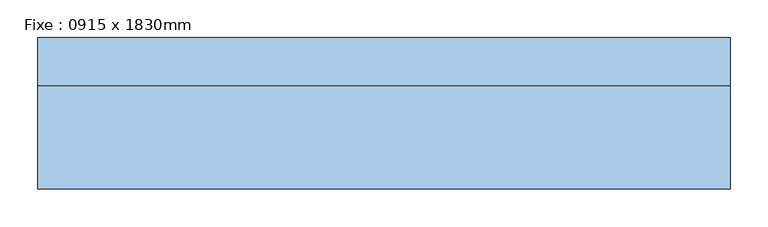
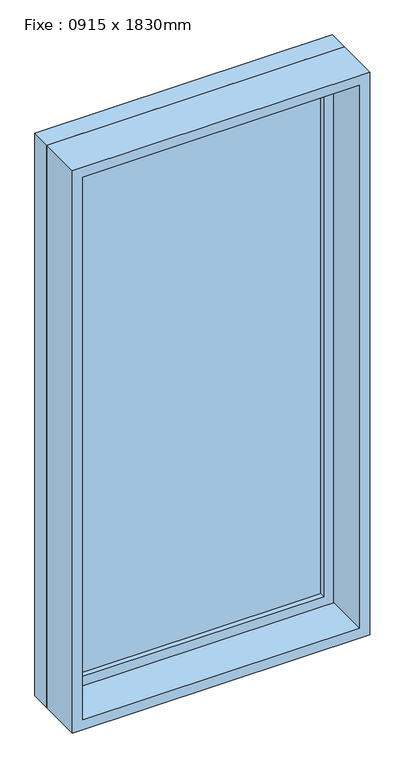
"""IFC4 building model written with IfcOpenShell, lengths in millimetres: window geometry, Fixe : 0915 x 1830mm."""

import ifcopenshell
import ifcopenshell.guid

model = None  # the IFC model being written
_history = None  # IfcOwnerHistory: only IFC2X3 demands one
_inside = {}  # id of a spatial element -> (the spatial element, [elements in it])
_under = {}  # id of a project, library or spatial element -> (it, [spatial elements below it])
_declared = {}  # id of a project -> (the project, [libraries it declares])
_typed = {}  # id of a type object -> (the type object, [elements of that type])
_made_of = {}  # id of a material, layer set ... -> (it, [elements and type objects made of it])


def new_model(schema):
    """Start an empty IFC model of exactly this schema.

    Asked for "IFC4X3", IfcOpenShell would pick the latest addendum, in which some entities
    have other attributes; the version numbers below select the first issue.
    IFC2X3 requires an IfcOwnerHistory on every rooted entity: one is made here for all.
    """
    global model, _history
    if schema == "IFC4X3":
        model = ifcopenshell.file(schema_version=(4, 3, 0, 0))
    else:
        model = ifcopenshell.file(schema=schema)
    _inside.clear()
    _under.clear()
    _declared.clear()
    _typed.clear()
    _made_of.clear()
    _history = None
    if model.schema == "IFC2X3":
        org = make("IfcOrganization", Name="unknown")
        user = make(
            "IfcPersonAndOrganization",
            ThePerson=make("IfcPerson", FamilyName="unknown"),
            TheOrganization=org,
        )
        app = make(
            "IfcApplication",
            ApplicationDeveloper=org,
            Version="unknown",
            ApplicationFullName="unknown",
            ApplicationIdentifier="unknown",
        )
        _history = make(
            "IfcOwnerHistory",
            OwningUser=user,
            OwningApplication=app,
            ChangeAction="ADDED",
            CreationDate=0,
        )
    return model


def make(cls, **values):
    """One entity of the class cls with the attributes given. An attribute that is None is left unset."""
    return model.create_entity(
        cls, **{name: value for name, value in values.items() if value is not None}
    )


def rooted(cls, **values):
    """An entity with a GlobalId (a new one), such as an element, a storey or a relation."""
    return make(cls, GlobalId=ifcopenshell.guid.new(), OwnerHistory=_history, **values)


def si_unit(unit_type, name, prefix=None):
    """IfcSIUnit, for example si_unit("LENGTHUNIT", "METRE", prefix="MILLI")."""
    return make("IfcSIUnit", UnitType=unit_type, Prefix=prefix, Name=name)


def assignment(units):
    """IfcUnitAssignment: the units of a project."""
    return None if units is None else make("IfcUnitAssignment", Units=units)


def point(xyz):
    """IfcCartesianPoint."""
    return None if xyz is None else make("IfcCartesianPoint", Coordinates=xyz)


def direction(xyz):
    """IfcDirection."""
    return None if xyz is None else make("IfcDirection", DirectionRatios=xyz)


def frame(location, z_axis=None, x_axis=None):
    """IfcAxis2Placement3D, a coordinate frame: its origin and axes. An axis left out is left unset."""
    return make(
        "IfcAxis2Placement3D",
        Location=point(location),
        Axis=direction(z_axis),
        RefDirection=direction(x_axis),
    )


def origin():
    """The frame at (0, 0, 0) with its axes left unset."""
    return frame((0.0, 0.0, 0.0))


def place(relative_to, where):
    """IfcLocalPlacement: puts the frame where relative to a parent placement (None: the world)."""
    return make(
        "IfcLocalPlacement", PlacementRelTo=relative_to, RelativePlacement=where
    )


def context(
    kind, dimensions, precision=None, world=None, true_north=None, identifier=None
):
    """IfcGeometricRepresentationContext, for example the 3D "Model" context."""
    return make(
        "IfcGeometricRepresentationContext",
        ContextIdentifier=identifier,
        ContextType=kind,
        CoordinateSpaceDimension=dimensions,
        Precision=precision,
        WorldCoordinateSystem=world,
        TrueNorth=true_north,
    )


def project(units=None, contexts=None):
    """IfcProject with its units and contexts."""
    return rooted(
        "IfcProject",
        Name="project",
        RepresentationContexts=contexts,
        UnitsInContext=assignment(units),
    )


def spatial(cls, under=None, at=None, **own):
    """A site, building, storey or space (cls), placed at a placement, below another one or the project."""
    s = rooted(cls, ObjectPlacement=at, **own)
    if under is not None:
        _under.setdefault(under.id(), (under, []))[1].append(s)
    return s


def polyline(points):
    """IfcPolyline through the points."""
    return make("IfcPolyline", Points=[point(p) for p in points])


def outline(outer, holes=None, kind="AREA"):
    """IfcArbitraryClosedProfileDef: a profile drawn as a closed curve; with holes, ...WithVoids."""
    if holes is None:
        return make("IfcArbitraryClosedProfileDef", ProfileType=kind, OuterCurve=outer)
    return make(
        "IfcArbitraryProfileDefWithVoids",
        ProfileType=kind,
        OuterCurve=outer,
        InnerCurves=holes,
    )


def extrude(swept, where, along, depth):
    """IfcExtrudedAreaSolid: the profile swept, set in the frame where, extruded along a direction by depth."""
    return make(
        "IfcExtrudedAreaSolid",
        SweptArea=swept,
        Position=where,
        ExtrudedDirection=direction(along),
        Depth=depth,
    )


def shape(context_of_items, identifier, shape_type, items):
    """IfcShapeRepresentation: the items that make up one representation, for example the "Body"."""
    return make(
        "IfcShapeRepresentation",
        ContextOfItems=context_of_items,
        RepresentationIdentifier=identifier,
        RepresentationType=shape_type,
        Items=items,
    )


def source(mapping_origin, context_of_items, identifier, shape_type, items):
    """IfcRepresentationMap: a shape defined once, which mapped items show again and again."""
    return make(
        "IfcRepresentationMap",
        MappingOrigin=mapping_origin,
        MappedRepresentation=shape(context_of_items, identifier, shape_type, items),
    )


def transform(
    local_origin,
    x_axis=None,
    y_axis=None,
    z_axis=None,
    scale=None,
    scale2=None,
    scale3=None,
    uniform=True,
):
    """IfcCartesianTransformationOperator3D, or its non-uniform kind. x_axis, y_axis, z_axis: its Axis1, 2, 3."""
    if uniform:
        return make(
            "IfcCartesianTransformationOperator3D",
            Axis1=direction(x_axis),
            Axis2=direction(y_axis),
            LocalOrigin=point(local_origin),
            Scale=scale,
            Axis3=direction(z_axis),
        )
    return make(
        "IfcCartesianTransformationOperator3DnonUniform",
        Axis1=direction(x_axis),
        Axis2=direction(y_axis),
        LocalOrigin=point(local_origin),
        Scale=scale,
        Axis3=direction(z_axis),
        Scale2=scale2,
        Scale3=scale3,
    )


def mapped(mapping_source, mapping_target):
    """IfcMappedItem: shows the shape of a source again, moved by a transform."""
    return make(
        "IfcMappedItem", MappingSource=mapping_source, MappingTarget=mapping_target
    )


def made_of(thing, what):
    """Note that an element or type object is made of a material, layer set ...; save() writes the relation."""
    if what is not None:
        _made_of.setdefault(what.id(), (what, []))[1].append(thing)
    return thing


def element(
    cls,
    number,
    at=None,
    inside=None,
    cuts=None,
    type_object=None,
    material=None,
    context=None,
    identifier="Body",
    shape_type=None,
    held_by="IfcProductDefinitionShape",
    body=None,
    shapes=None,
    **own,
):
    """One element of the class cls, such as IfcWall. Its Tag is "e" and its number.

    at: its placement. inside: the storey or other place that contains it. cuts: it is an
    opening in that element (IfcRelVoidsElement). A single representation is given by context,
    identifier, shape_type and body (its items); several are given by shapes. held_by: the class
    of the entity that holds the representations. save() writes the other relations.
    """
    e = rooted(cls, Tag="e%d" % number, ObjectPlacement=at, **own)
    if body is not None:
        shapes = [shape(context, identifier, shape_type, body)]
    if shapes is not None:
        e.Representation = make(held_by, Representations=shapes)
    if inside is not None:
        _inside.setdefault(inside.id(), (inside, []))[1].append(e)
    if cuts is not None:
        rooted(
            "IfcRelVoidsElement", RelatingBuildingElement=cuts, RelatedOpeningElement=e
        )
    if type_object is not None:
        _typed.setdefault(type_object.id(), (type_object, []))[1].append(e)
    return made_of(e, material)


def aggregate(whole, parts):
    """IfcRelAggregates: a whole, such as a stair, and the parts it consists of."""
    return rooted("IfcRelAggregates", RelatingObject=whole, RelatedObjects=parts)


def save(model, path):
    """Write the relations noted so far, then the file.

    IfcRelAggregates (storeys below a building ...), IfcRelContainedInSpatialStructure (elements
    in a storey), IfcRelDefinesByType, IfcRelAssociatesMaterial and IfcRelDeclares: one each for
    every whole, place, type object, material and project.
    """
    for whole, parts in _under.values():
        aggregate(whole, parts)
    for where, things in _inside.values():
        rooted(
            "IfcRelContainedInSpatialStructure",
            RelatedElements=things,
            RelatingStructure=where,
        )
    for kind, things in _typed.values():
        rooted("IfcRelDefinesByType", RelatedObjects=things, RelatingType=kind)
    for what, things in _made_of.values():
        rooted("IfcRelAssociatesMaterial", RelatedObjects=things, RelatingMaterial=what)
    for by, libraries in _declared.values():
        rooted("IfcRelDeclares", RelatingContext=by, RelatedDefinitions=libraries)
    model.write(path)


def fixe_0915_x_1830mm_5d6e8bc1(model_context):
    return source(origin(), model_context, "Body", "SweptSolid", [
        extrude(outline(polyline([(-394.5, 78.0), (394.5, 78.0), (394.5, 66.0), (-394.5, 66.0), (-394.5, 78.0)])), frame((0.0, 0.0, 368.0), z_axis=(0.0, 0.0, 1.0), x_axis=(1.0, 0.0, 0.0)), (0.0, 0.0, 1.0), 1704.0),
        extrude(outline(polyline([(2116.0, -438.5), (324.0, -438.5), (324.0, 438.5), (2116.0, 438.5), (2116.0, -438.5)]), holes=[polyline([(2072.0, -394.5), (2072.0, 394.5), (368.0, 394.5), (368.0, -394.5), (2072.0, -394.5)])]), frame((0.0, 50.0, 0.0), z_axis=(0.0, 1.0, 0.0), x_axis=(0.0, 0.0, 1.0)), (0.0, 0.0, 1.0), 44.0),
        extrude(outline(polyline([(2135.0, -457.5), (305.0, -457.5), (305.0, 457.5), (2135.0, 457.5), (2135.0, -457.5)]), holes=[polyline([(2116.0, -438.5), (2116.0, 438.5), (324.0, 438.5), (324.0, -438.5), (2116.0, -438.5)])]), frame((0.0, 50.0, 0.0), z_axis=(0.0, 1.0, 0.0), x_axis=(0.0, 0.0, 1.0)), (0.0, 0.0, 1.0), 63.0),
        extrude(outline(polyline([(2135.0, -457.5), (305.0, -457.5), (305.0, 457.5), (2135.0, 457.5), (2135.0, -457.5)]), holes=[polyline([(2103.0, -425.5), (2103.0, 425.5), (337.0, 425.5), (337.0, -425.5), (2103.0, -425.5)])]), frame((0.0, -87.0, 0.0), z_axis=(0.0, 1.0, 0.0), x_axis=(0.0, 0.0, 1.0)), (0.0, 0.0, 1.0), 137.0),
    ])


if __name__ == "__main__":
    model = new_model("IFC4")
    model_context = context("Model", 3, world=origin())
    ifc_project = project(units=[si_unit("LENGTHUNIT", "METRE", prefix="MILLI")], contexts=[model_context])
    site = spatial("IfcSite", under=ifc_project)
    building = spatial("IfcBuilding", under=site)
    placement = place(None, origin())
    fixe_0915_x_1830mm_shape = fixe_0915_x_1830mm_5d6e8bc1(model_context)
    element("IfcWindow", 1, ObjectType="Fixe : 0915 x 1830mm", at=placement, inside=building, context=model_context, shape_type="MappedRepresentation", body=[
        mapped(fixe_0915_x_1830mm_shape, transform((0.0, 0.0, 0.0), x_axis=(1.0, 0.0, 0.0), y_axis=(0.0, 1.0, 0.0), z_axis=(0.0, 0.0, 1.0))),
    ])
    save(model, "model.ifc")

# Revit data of these elements
# Type "Fixe : 0915 x 1830mm"
#   Type Mark = "18"
#   Construction Type Id = "GSP4R"
#   Analytic Construction = "Simple vitrage Pilkington 1/8 po."
#   Visual Light Transmittance = 0.9
#   Solar Heat Gain Coefficient = 0.78
#   Heat Transfer Coefficient (U) = 3.6886 W/(m²·K)
#   Height = 1.83 m
#   Hauteur de l'appui par défaut = 0.305 m
#   Width = 0.915 m
#   Encastrement de fenêtre = 0.019 m
#   Define Thermal Properties by = 1
#   Matériau de cadre extérieur = Châssis
#   Matériau du cadre intérieur = Châssis
#   Matériau du panneau de verre = Verre
#   Châssis = Châssis
#   Wall Closure = (empty or 0)
# Element 1 (IfcWindow, "Fixe : 0915 x 1830mm")
#   Materials on its faces: "Châssis", "Verre"
# Materials
#   "Châssis": class "Bois", colour RGB 224 178 126, transparency 0, Cost = 0
#   "Verre": class "Verre", colour RGB 0 128 192, transparency 0.9, Description = "Verre sodocalcique", Cost = 0
